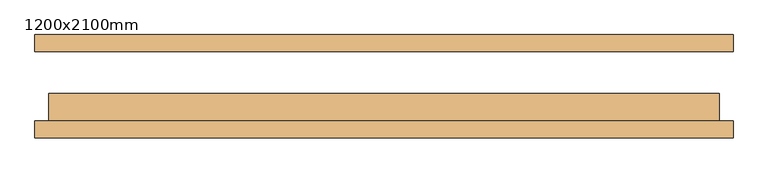
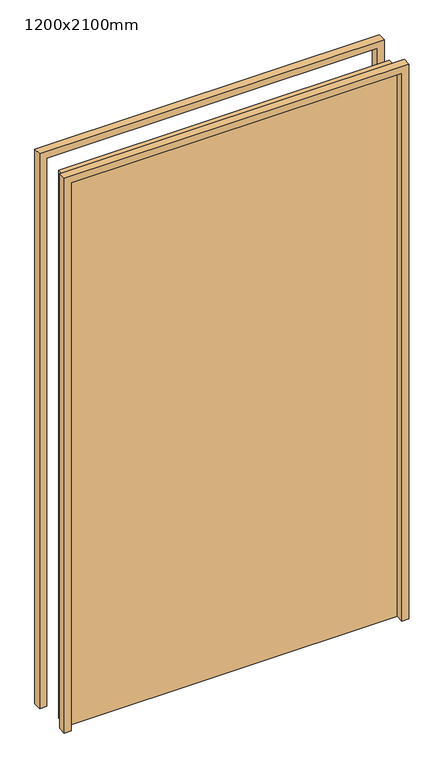
"""IFC4 building model written with IfcOpenShell, lengths in millimetres: door geometry, WWm-SingleSolid-Flush : 1200x2100mm."""

from ifc_helpers import new_model, si_unit, frame, origin, origin_with_axes, place, context, project, spatial, polyline, outline, extrude, source, transform, mapped, element, save


def door_1200x2100mm_cbea3ea0(model_context):
    return source(origin(), model_context, "Body", "SweptSolid", [
        extrude(outline(polyline([(2125.0, -625.0), (0.0, -625.0), (0.0, -600.0), (2100.0, -600.0), (2100.0, 600.0), (0.0, 600.0), (0.0, 625.0), (2125.0, 625.0), (2125.0, -625.0)])), frame((0.0, -92.5, 0.0), z_axis=(0.0, 1.0, 0.0), x_axis=(0.0, 0.0, 1.0)), (0.0, 0.0, 1.0), 30.0),
        extrude(outline(polyline([(2125.0, 625.0), (2125.0, -625.0), (0.0, -625.0), (0.0, -600.0), (2100.0, -600.0), (2100.0, 600.0), (0.0, 600.0), (0.0, 625.0), (2125.0, 625.0)])), frame((0.0, 62.5, 0.0), z_axis=(0.0, 1.0, 0.0), x_axis=(0.0, 0.0, 1.0)), (0.0, 0.0, 1.0), 30.0),
        extrude(outline(polyline([(600.0, -12.5), (600.0, -62.5), (-600.0, -62.5), (-600.0, -12.5), (600.0, -12.5)])), origin_with_axes(), (0.0, 0.0, 1.0), 2100.0),
    ])


if __name__ == "__main__":
    model = new_model("IFC4")
    model_context = context("Model", 3, world=origin())
    ifc_project = project(units=[si_unit("LENGTHUNIT", "METRE", prefix="MILLI")], contexts=[model_context])
    site = spatial("IfcSite", under=ifc_project)
    building = spatial("IfcBuilding", under=site)
    placement = place(None, origin())
    door_1200x2100mm_shape = door_1200x2100mm_cbea3ea0(model_context)
    element("IfcDoor", 1, ObjectType="WWm-SingleSolid-Flush : 1200x2100mm", at=placement, inside=building, context=model_context, shape_type="MappedRepresentation", body=[
        mapped(door_1200x2100mm_shape, transform((0.0, 0.0, 0.0), x_axis=(1.0, 0.0, 0.0), y_axis=(0.0, 1.0, 0.0), z_axis=(0.0, 0.0, 1.0))),
    ])
    save(model, "model.ifc")

# Revit data of these elements
# Type "WWm-SingleSolid-Flush : 1200x2100mm"
#   Type Mark = "EX1-55"
#   Construction Type Id = "MDOOR"
#   Assembly Code = "C1020"
#   Analytic Construction = "Metal"
#   Thickness = 50 mm
#   Thermal Resistance (R) = 0.270117 (m²·K)/W
#   Heat Transfer Coefficient (U) = 3.7021 W/(m²·K)
#   Height = 2100 mm
#   Trim Projection Ext = 30 mm
#   Trim Projection Int = 30 mm
#   Trim Width = 25 mm
#   Width = 1200 mm
#   Not 90 Degree [instance default] = no
#   90 Degree [instance default] = yes
#   Door Material = WW-EC-RGB-White
#   Frame Material = WW-EC-RGB-White
#   Visual Light Transmittance = 0
#   Solar Heat Gain Coefficient = 0
#   Function = (empty or 0)
#   Wall Closure = (empty or 0)
# Element 1 (IfcDoor, "WWm-SingleSolid-Flush : 1200x2100mm")
#   Materials on its faces: "WW-EC-RGB-White"
# Materials
#   "WW-EC-RGB-White": class "Generic", colour RGB 255 255 255, transparency 0, Comments = "If region requests off-white, swith asset color to RGB 231-228-220", Description = "Generic Color", Cost = 0
